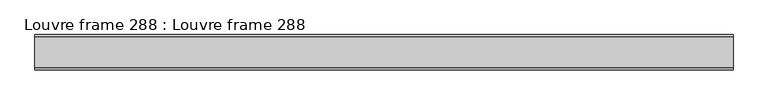
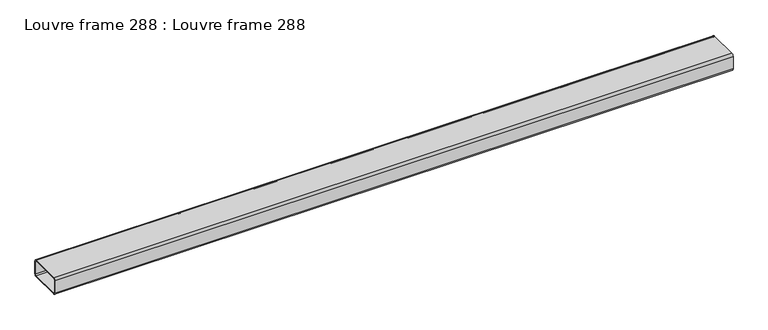
"""IFC4 building model written with IfcOpenShell, lengths in millimetres: proxy geometry, Louvre frame 288 : Louvre frame 288."""

from ifc_helpers import new_model, si_unit, point, frame, frame_2d, origin, place, context, project, spatial, polyline, circle_curve, trimmed, segment, composite_curve, outline, extrude, source, transform, mapped, element, save


def louvre_frame_288_louvre_frame_288_dedd44c9(model_context):
    return source(origin(), model_context, "Body", "SweptSolid", [
        extrude(outline(composite_curve([segment(trimmed(circle_curve(frame_2d((9795.5719584, 39482.0859375)), 6.35), [point((9795.5719584, 39475.7359375))], [point((9789.2219584, 39482.0859375))], False, "CARTESIAN"), True, "CONTINUOUS"), segment(polyline([(9789.2219584, 39482.0859375), (9789.2219584, 39520.1859375)]), True, "CONTINUOUS"), segment(trimmed(circle_curve(frame_2d((9795.5719584, 39520.1859375)), 6.35), [point((9789.2219584, 39520.1859375))], [point((9795.5719584, 39526.5359375))], False, "CARTESIAN"), True, "CONTINUOUS"), segment(polyline([(9795.5719584, 39526.5359375), (9884.4719584, 39526.5359375)]), True, "CONTINUOUS"), segment(trimmed(circle_curve(frame_2d((9884.4719584, 39520.1859375)), 6.35), [point((9884.4719584, 39526.5359375))], [point((9890.8219584, 39520.1859375))], False, "CARTESIAN"), True, "CONTINUOUS"), segment(polyline([(9890.8219584, 39520.1859375), (9890.8219584, 39482.0859375)]), True, "CONTINUOUS"), segment(trimmed(circle_curve(frame_2d((9884.4719584, 39482.0859375)), 6.35), [point((9890.8219584, 39482.0859375))], [point((9884.4719584, 39475.7359375))], False, "CARTESIAN"), True, "CONTINUOUS"), segment(polyline([(9884.4719584, 39475.7359375), (9795.5719584, 39475.7359375)]), True, "CONTINUOUS")], self_intersect=False), holes=[composite_curve([segment(polyline([(9887.6519584, 39482.0859375), (9887.6519584, 39520.1859375)]), True, "CONTINUOUS"), segment(trimmed(circle_curve(frame_2d((9884.4719584, 39520.1859375)), 3.18), [point((9887.6519584, 39520.1859375))], [point((9884.4719584, 39523.3659375))], True, "CARTESIAN"), True, "CONTINUOUS"), segment(polyline([(9884.4719584, 39523.3659375), (9795.5719584, 39523.3659375)]), True, "CONTINUOUS"), segment(trimmed(circle_curve(frame_2d((9795.5719584, 39520.1859375)), 3.18), [point((9795.5719584, 39523.3659375))], [point((9792.3919584, 39520.1859375))], True, "CARTESIAN"), True, "CONTINUOUS"), segment(polyline([(9792.3919584, 39520.1859375), (9792.3919584, 39482.0859375)]), True, "CONTINUOUS"), segment(trimmed(circle_curve(frame_2d((9795.5719584, 39482.0859375)), 3.18), [point((9792.3919584, 39482.0859375))], [point((9795.5719584, 39478.9059375))], True, "CARTESIAN"), True, "CONTINUOUS"), segment(polyline([(9795.5719584, 39478.9059375), (9884.4719584, 39478.9059375)]), True, "CONTINUOUS"), segment(trimmed(circle_curve(frame_2d((9884.4719584, 39482.0859375)), 3.18), [point((9884.4719584, 39478.9059375))], [point((9887.6519584, 39482.0859375))], True, "CARTESIAN"), True, "CONTINUOUS")], self_intersect=False)]), frame((3694.2883192, 0.0, 0.0), z_axis=(1.0, 0.0, 0.0), x_axis=(0.0, 1.0, 0.0)), (0.0, 0.0, 1.0), 2000.0),
    ])


if __name__ == "__main__":
    model = new_model("IFC4")
    model_context = context("Model", 3, world=origin())
    ifc_project = project(units=[si_unit("LENGTHUNIT", "METRE", prefix="MILLI")], contexts=[model_context])
    site = spatial("IfcSite", under=ifc_project)
    building = spatial("IfcBuilding", under=site)
    placement = place(None, origin())
    louvre_frame_288_louvre_frame_288_shape = louvre_frame_288_louvre_frame_288_dedd44c9(model_context)
    element("IfcBuildingElementProxy", 1, Name="Louvre frame 288 : Louvre frame 288", ObjectType="Louvre frame 288 : Louvre frame 288", at=placement, inside=building, context=model_context, shape_type="MappedRepresentation", body=[
        mapped(louvre_frame_288_louvre_frame_288_shape, transform((0.0, 0.0, 0.0), x_axis=(1.0, 0.0, 0.0), y_axis=(0.0, 1.0, 0.0), z_axis=(0.0, 0.0, 1.0))),
    ])
    save(model, "model.ifc")

# Revit data of these elements
# Type "Louvre frame 288 : Louvre frame 288"
#   NameOverride = "Louvre frame"
# Element 1 (IfcBuildingElementProxy, "Louvre frame 288 : Louvre frame 288")
#   Materials on its faces: "ALUMINIUM LOUVRE - TBD"
# Materials
#   "ALUMINIUM LOUVRE - TBD": class "Unassigned", colour RGB 92 107 122, transparency 0
